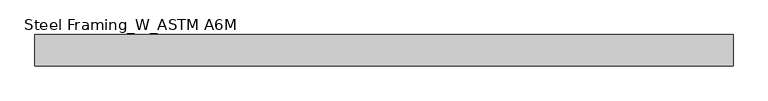
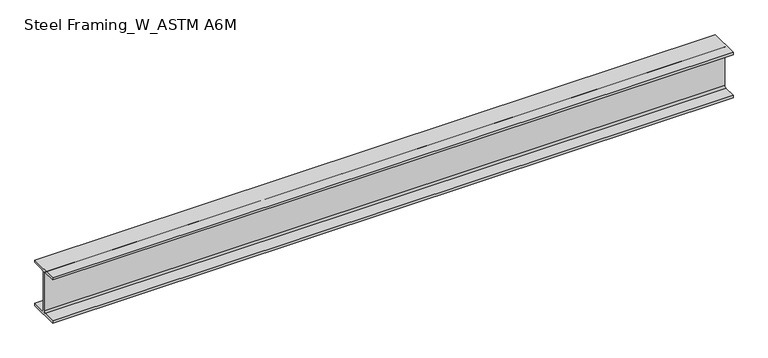
"""IFC4 building model written with IfcOpenShell, lengths in millimetres: beam geometry, Steel Framing_W_ASTM A6M : H_SB_AR_S02_W200x31.3_RB4."""

from ifc_helpers import new_model, si_unit, point, frame, frame_2d, origin, place, context, project, spatial, polyline, circle_curve, trimmed, segment, composite_curve, outline, extrude, source, transform, mapped, element, save


def steel_framing_w_astm_a6m_278bd3b7(model_context):
    return source(origin(), model_context, "Body", "SweptSolid", [
        extrude(outline(composite_curve([segment(polyline([(67.0, -94.8), (67.0, -105.0), (-67.0, -105.0), (-67.0, -94.8), (-10.775, -94.8)]), True, "CONTINUOUS"), segment(trimmed(circle_curve(frame_2d((-10.775, -87.2)), 7.6), [point((-10.775, -94.8))], [point((-3.175, -87.2))], True, "CARTESIAN"), True, "CONTINUOUS"), segment(polyline([(-3.175, -87.2), (-3.175, 87.2)]), True, "CONTINUOUS"), segment(trimmed(circle_curve(frame_2d((-10.775, 87.2)), 7.6), [point((-3.175, 87.2))], [point((-10.775, 94.8))], True, "CARTESIAN"), True, "CONTINUOUS"), segment(polyline([(-10.775, 94.8), (-67.0, 94.8), (-67.0, 105.0), (67.0, 105.0), (67.0, 94.8), (10.775, 94.8)]), True, "CONTINUOUS"), segment(trimmed(circle_curve(frame_2d((10.775, 87.2)), 7.6), [point((10.775, 94.8))], [point((3.175, 87.2))], True, "CARTESIAN"), True, "CONTINUOUS"), segment(polyline([(3.175, 87.2), (3.175, -87.2)]), True, "CONTINUOUS"), segment(trimmed(circle_curve(frame_2d((10.775, -87.2)), 7.6), [point((3.175, -87.2))], [point((10.775, -94.8))], True, "CARTESIAN"), True, "CONTINUOUS"), segment(polyline([(10.775, -94.8), (67.0, -94.8)]), True, "CONTINUOUS")], self_intersect=False)), frame((-1500.0, 0.0, 0.0), z_axis=(1.0, 0.0, 0.0), x_axis=(0.0, 1.0, 0.0)), (0.0, 0.0, 1.0), 2987.2),
    ])


if __name__ == "__main__":
    model = new_model("IFC4")
    model_context = context("Model", 3, world=origin())
    ifc_project = project(units=[si_unit("LENGTHUNIT", "METRE", prefix="MILLI")], contexts=[model_context])
    site = spatial("IfcSite", under=ifc_project)
    building = spatial("IfcBuilding", under=site)
    placement = place(None, origin())
    steel_framing_w_astm_a6m_shape = steel_framing_w_astm_a6m_278bd3b7(model_context)
    element("IfcBeam", 1, ObjectType="Steel Framing_W_ASTM A6M : H_SB_AR_S02_W200x31.3_RB4", at=placement, inside=building, context=model_context, shape_type="MappedRepresentation", body=[
        mapped(steel_framing_w_astm_a6m_shape, transform((0.0, 0.0, 0.0), x_axis=(1.0, 0.0, 0.0), y_axis=(0.0, 1.0, 0.0), z_axis=(0.0, 0.0, 1.0))),
    ])
    save(model, "model.ifc")

# Revit data of these elements
# Type "Steel Framing_W_ASTM A6M : H_SB_AR_S02_W200x31.3_RB4"
#   Type Mark = "RB4"
#   Section Name Key = "W8x21"
#   Width = 13.4 cm
#   Web Thickness = 0.635 cm
#   Web Fillet = 0.76 cm
#   Warping Constant = 40800.0 cm⁶
#   Torsional Moment of Inertia = 11.70 cm⁴
#   Section Area = 39.7 cm²
#   Plastic Modulus weak axis = 93.2 cm³
#   Plastic Modulus strong axis = 334.0 cm³
#   Perimeter = 0.93 m²/m
#   Nominal Weight = 31.30 kgf/m
#   Moment of Inertia weak axis = 407.00 cm⁴
#   Moment of Inertia strong axis = 3130.00 cm⁴
#   Height = 21.0 cm
#   Flange Thickness = 1.02 cm
#   Elastic Modulus weak axis = 60.8 cm³
#   Elastic Modulus strong axis = 298.0 cm³
#   Centroid Vertical = 10.5 cm
#   Centroid Horizontal = 6.7 cm
#   Length [instance default] = 1500 mm
#   Structural Material [instance default] = Steel, 45-345
#   Bolt Spacing = 0
#   Assembly Code = ""
# Element 1 (IfcBeam, "Steel Framing_W_ASTM A6M : H_SB_AR_S02_W200x31.3_RB4")
#   Materials on its faces: "Steel, 45-345"
# Materials
#   "Steel, 45-345": class "Metal", colour RGB 189 187 185, transparency 0, Description = "Steel 345 MPa", Cost = 0
